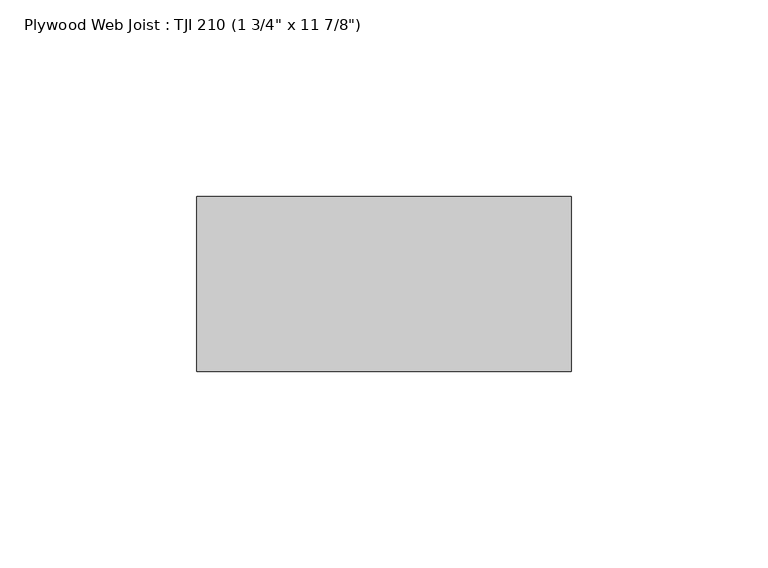
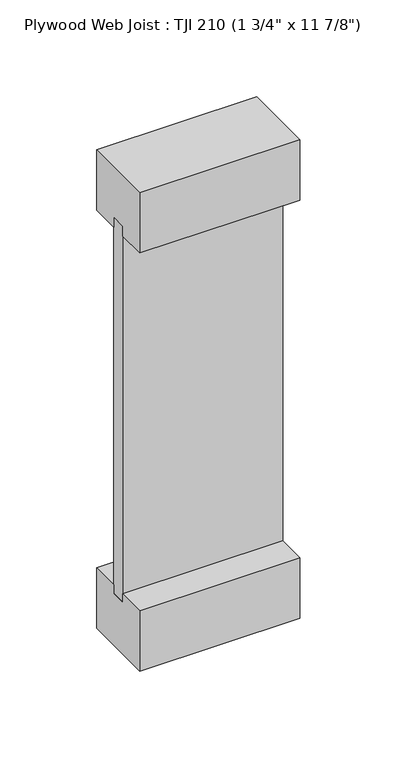
"""IFC4 building model written with IfcOpenShell, lengths in millimetres: beam geometry."""

import ifcopenshell
import ifcopenshell.guid

model = None  # the IFC model being written
_history = None  # IfcOwnerHistory: only IFC2X3 demands one
_inside = {}  # id of a spatial element -> (the spatial element, [elements in it])
_under = {}  # id of a project, library or spatial element -> (it, [spatial elements below it])
_declared = {}  # id of a project -> (the project, [libraries it declares])
_typed = {}  # id of a type object -> (the type object, [elements of that type])
_made_of = {}  # id of a material, layer set ... -> (it, [elements and type objects made of it])


def new_model(schema):
    """Start an empty IFC model of exactly this schema.

    Asked for "IFC4X3", IfcOpenShell would pick the latest addendum, in which some entities
    have other attributes; the version numbers below select the first issue.
    IFC2X3 requires an IfcOwnerHistory on every rooted entity: one is made here for all.
    """
    global model, _history
    if schema == "IFC4X3":
        model = ifcopenshell.file(schema_version=(4, 3, 0, 0))
    else:
        model = ifcopenshell.file(schema=schema)
    _inside.clear()
    _under.clear()
    _declared.clear()
    _typed.clear()
    _made_of.clear()
    _history = None
    if model.schema == "IFC2X3":
        org = make("IfcOrganization", Name="unknown")
        user = make(
            "IfcPersonAndOrganization",
            ThePerson=make("IfcPerson", FamilyName="unknown"),
            TheOrganization=org,
        )
        app = make(
            "IfcApplication",
            ApplicationDeveloper=org,
            Version="unknown",
            ApplicationFullName="unknown",
            ApplicationIdentifier="unknown",
        )
        _history = make(
            "IfcOwnerHistory",
            OwningUser=user,
            OwningApplication=app,
            ChangeAction="ADDED",
            CreationDate=0,
        )
    return model


def make(cls, **values):
    """One entity of the class cls with the attributes given. An attribute that is None is left unset."""
    return model.create_entity(
        cls, **{name: value for name, value in values.items() if value is not None}
    )


def rooted(cls, **values):
    """An entity with a GlobalId (a new one), such as an element, a storey or a relation."""
    return make(cls, GlobalId=ifcopenshell.guid.new(), OwnerHistory=_history, **values)


def si_unit(unit_type, name, prefix=None):
    """IfcSIUnit, for example si_unit("LENGTHUNIT", "METRE", prefix="MILLI")."""
    return make("IfcSIUnit", UnitType=unit_type, Prefix=prefix, Name=name)


def assignment(units):
    """IfcUnitAssignment: the units of a project."""
    return None if units is None else make("IfcUnitAssignment", Units=units)


def point(xyz):
    """IfcCartesianPoint."""
    return None if xyz is None else make("IfcCartesianPoint", Coordinates=xyz)


def direction(xyz):
    """IfcDirection."""
    return None if xyz is None else make("IfcDirection", DirectionRatios=xyz)


def frame(location, z_axis=None, x_axis=None):
    """IfcAxis2Placement3D, a coordinate frame: its origin and axes. An axis left out is left unset."""
    return make(
        "IfcAxis2Placement3D",
        Location=point(location),
        Axis=direction(z_axis),
        RefDirection=direction(x_axis),
    )


def origin():
    """The frame at (0, 0, 0) with its axes left unset."""
    return frame((0.0, 0.0, 0.0))


def place(relative_to, where):
    """IfcLocalPlacement: puts the frame where relative to a parent placement (None: the world)."""
    return make(
        "IfcLocalPlacement", PlacementRelTo=relative_to, RelativePlacement=where
    )


def context(
    kind, dimensions, precision=None, world=None, true_north=None, identifier=None
):
    """IfcGeometricRepresentationContext, for example the 3D "Model" context."""
    return make(
        "IfcGeometricRepresentationContext",
        ContextIdentifier=identifier,
        ContextType=kind,
        CoordinateSpaceDimension=dimensions,
        Precision=precision,
        WorldCoordinateSystem=world,
        TrueNorth=true_north,
    )


def project(units=None, contexts=None):
    """IfcProject with its units and contexts."""
    return rooted(
        "IfcProject",
        Name="project",
        RepresentationContexts=contexts,
        UnitsInContext=assignment(units),
    )


def spatial(cls, under=None, at=None, **own):
    """A site, building, storey or space (cls), placed at a placement, below another one or the project."""
    s = rooted(cls, ObjectPlacement=at, **own)
    if under is not None:
        _under.setdefault(under.id(), (under, []))[1].append(s)
    return s


def polyline(points):
    """IfcPolyline through the points."""
    return make("IfcPolyline", Points=[point(p) for p in points])


def outline(outer, holes=None, kind="AREA"):
    """IfcArbitraryClosedProfileDef: a profile drawn as a closed curve; with holes, ...WithVoids."""
    if holes is None:
        return make("IfcArbitraryClosedProfileDef", ProfileType=kind, OuterCurve=outer)
    return make(
        "IfcArbitraryProfileDefWithVoids",
        ProfileType=kind,
        OuterCurve=outer,
        InnerCurves=holes,
    )


def extrude(swept, where, along, depth):
    """IfcExtrudedAreaSolid: the profile swept, set in the frame where, extruded along a direction by depth."""
    return make(
        "IfcExtrudedAreaSolid",
        SweptArea=swept,
        Position=where,
        ExtrudedDirection=direction(along),
        Depth=depth,
    )


def shape(context_of_items, identifier, shape_type, items):
    """IfcShapeRepresentation: the items that make up one representation, for example the "Body"."""
    return make(
        "IfcShapeRepresentation",
        ContextOfItems=context_of_items,
        RepresentationIdentifier=identifier,
        RepresentationType=shape_type,
        Items=items,
    )


def source(mapping_origin, context_of_items, identifier, shape_type, items):
    """IfcRepresentationMap: a shape defined once, which mapped items show again and again."""
    return make(
        "IfcRepresentationMap",
        MappingOrigin=mapping_origin,
        MappedRepresentation=shape(context_of_items, identifier, shape_type, items),
    )


def transform(
    local_origin,
    x_axis=None,
    y_axis=None,
    z_axis=None,
    scale=None,
    scale2=None,
    scale3=None,
    uniform=True,
):
    """IfcCartesianTransformationOperator3D, or its non-uniform kind. x_axis, y_axis, z_axis: its Axis1, 2, 3."""
    if uniform:
        return make(
            "IfcCartesianTransformationOperator3D",
            Axis1=direction(x_axis),
            Axis2=direction(y_axis),
            LocalOrigin=point(local_origin),
            Scale=scale,
            Axis3=direction(z_axis),
        )
    return make(
        "IfcCartesianTransformationOperator3DnonUniform",
        Axis1=direction(x_axis),
        Axis2=direction(y_axis),
        LocalOrigin=point(local_origin),
        Scale=scale,
        Axis3=direction(z_axis),
        Scale2=scale2,
        Scale3=scale3,
    )


def mapped(mapping_source, mapping_target):
    """IfcMappedItem: shows the shape of a source again, moved by a transform."""
    return make(
        "IfcMappedItem", MappingSource=mapping_source, MappingTarget=mapping_target
    )


def made_of(thing, what):
    """Note that an element or type object is made of a material, layer set ...; save() writes the relation."""
    if what is not None:
        _made_of.setdefault(what.id(), (what, []))[1].append(thing)
    return thing


def element(
    cls,
    number,
    at=None,
    inside=None,
    cuts=None,
    type_object=None,
    material=None,
    context=None,
    identifier="Body",
    shape_type=None,
    held_by="IfcProductDefinitionShape",
    body=None,
    shapes=None,
    **own,
):
    """One element of the class cls, such as IfcWall. Its Tag is "e" and its number.

    at: its placement. inside: the storey or other place that contains it. cuts: it is an
    opening in that element (IfcRelVoidsElement). A single representation is given by context,
    identifier, shape_type and body (its items); several are given by shapes. held_by: the class
    of the entity that holds the representations. save() writes the other relations.
    """
    e = rooted(cls, Tag="e%d" % number, ObjectPlacement=at, **own)
    if body is not None:
        shapes = [shape(context, identifier, shape_type, body)]
    if shapes is not None:
        e.Representation = make(held_by, Representations=shapes)
    if inside is not None:
        _inside.setdefault(inside.id(), (inside, []))[1].append(e)
    if cuts is not None:
        rooted(
            "IfcRelVoidsElement", RelatingBuildingElement=cuts, RelatedOpeningElement=e
        )
    if type_object is not None:
        _typed.setdefault(type_object.id(), (type_object, []))[1].append(e)
    return made_of(e, material)


def aggregate(whole, parts):
    """IfcRelAggregates: a whole, such as a stair, and the parts it consists of."""
    return rooted("IfcRelAggregates", RelatingObject=whole, RelatedObjects=parts)


def save(model, path):
    """Write the relations noted so far, then the file.

    IfcRelAggregates (storeys below a building ...), IfcRelContainedInSpatialStructure (elements
    in a storey), IfcRelDefinesByType, IfcRelAssociatesMaterial and IfcRelDeclares: one each for
    every whole, place, type object, material and project.
    """
    for whole, parts in _under.values():
        aggregate(whole, parts)
    for where, things in _inside.values():
        rooted(
            "IfcRelContainedInSpatialStructure",
            RelatedElements=things,
            RelatingStructure=where,
        )
    for kind, things in _typed.values():
        rooted("IfcRelDefinesByType", RelatedObjects=things, RelatingType=kind)
    for what, things in _made_of.values():
        rooted("IfcRelAssociatesMaterial", RelatedObjects=things, RelatingMaterial=what)
    for by, libraries in _declared.values():
        rooted("IfcRelDeclares", RelatingContext=by, RelatedDefinitions=libraries)
    model.write(path)


def beam_e8d737f7(model_context):
    return source(origin(), model_context, "Body", "SweptSolid", [
        extrude(outline(polyline([(-22.225, 150.8125), (22.225, 150.8125), (22.225, 112.7125), (4.7625, 112.7125), (4.7625, 119.0625), (-4.7625, 119.0625), (-4.7625, 112.7125), (-22.225, 112.7125), (-22.225, 150.8125)])), frame((-84.1375, 0.0, 0.0), z_axis=(1.0, 0.0, 0.0), x_axis=(0.0, 1.0, 0.0)), (0.0, 0.0, 1.0), 95.25),
        extrude(outline(polyline([(22.225, -112.7125), (22.225, -150.8125), (-22.225, -150.8125), (-22.225, -112.7125), (-4.7625, -112.7125), (-4.7625, -118.3285374), (4.7625, -118.3285374), (4.7625, -112.7125), (22.225, -112.7125)])), frame((-84.1375, 0.0, 0.0), z_axis=(1.0, 0.0, 0.0), x_axis=(0.0, 1.0, 0.0)), (0.0, 0.0, 1.0), 95.25),
        extrude(outline(polyline([(11.1125, 4.7625), (11.1125, -4.7625), (-84.1375, -4.7625), (-84.1375, 4.7625), (11.1125, 4.7625)])), frame((0.0, 0.0, -118.3285374), z_axis=(0.0, 0.0, 1.0), x_axis=(1.0, 0.0, 0.0)), (0.0, 0.0, 1.0), 237.3910374),
    ])


if __name__ == "__main__":
    model = new_model("IFC4")
    model_context = context("Model", 3, world=origin())
    ifc_project = project(units=[si_unit("LENGTHUNIT", "METRE", prefix="MILLI")], contexts=[model_context])
    site = spatial("IfcSite", under=ifc_project)
    building = spatial("IfcBuilding", under=site)
    placement = place(None, origin())
    beam_shape = beam_e8d737f7(model_context)
    element("IfcBeam", 1, ObjectType="Plywood Web Joist : TJI 210 (1 3/4\" x 11 7/8\")", at=placement, inside=building, context=model_context, shape_type="MappedRepresentation", body=[
        mapped(beam_shape, transform((0.0, 0.0, 0.0), x_axis=(1.0, 0.0, 0.0), y_axis=(0.0, 1.0, 0.0), z_axis=(0.0, 0.0, 1.0))),
    ])
    save(model, "model.ifc")

# Revit data of these elements
# Type "Plywood Web Joist : TJI 210 (1 3/4\" x 11 7/8\")"
#   Assembly Code = "B10"
#   Length [instance default] = 5' - 0"
#   b = 0' - 1 3/4"
#   d = 0' - 11 7/8"
#   Structural Material [instance default] = Softwood, Lumber
# Element 1 (IfcBeam, "Plywood Web Joist : TJI 210 (1 3/4\" x 11 7/8\")")
#   Materials on its faces: "Softwood, Lumber"
# Materials
#   "Softwood, Lumber": class "Wood", colour RGB 144 113 62, transparency 0, Description = "Pinus Echinata", Cost = 0
